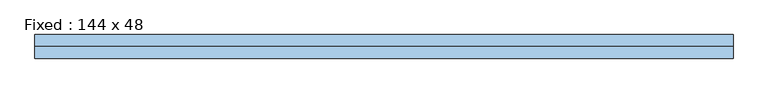
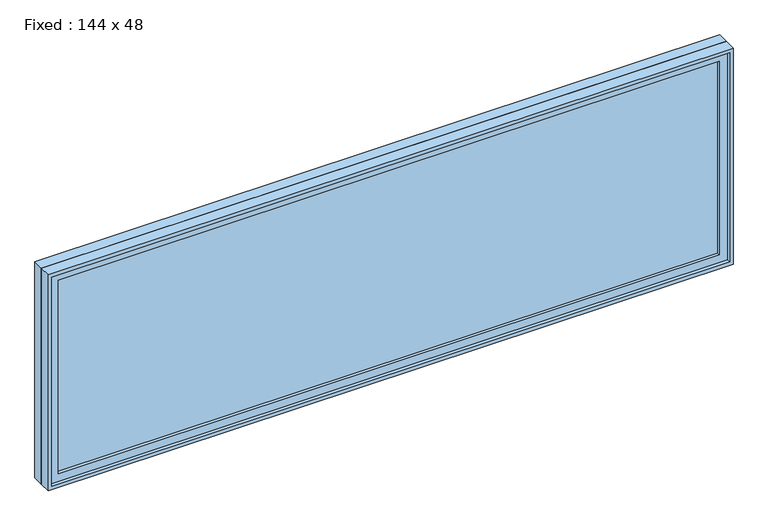
"""IFC4 building model written with IfcOpenShell, lengths in millimetres: window geometry, Fixed : 144 x 48."""

import ifcopenshell
import ifcopenshell.guid

model = None  # the IFC model being written
_history = None  # IfcOwnerHistory: only IFC2X3 demands one
_inside = {}  # id of a spatial element -> (the spatial element, [elements in it])
_under = {}  # id of a project, library or spatial element -> (it, [spatial elements below it])
_declared = {}  # id of a project -> (the project, [libraries it declares])
_typed = {}  # id of a type object -> (the type object, [elements of that type])
_made_of = {}  # id of a material, layer set ... -> (it, [elements and type objects made of it])


def new_model(schema):
    """Start an empty IFC model of exactly this schema.

    Asked for "IFC4X3", IfcOpenShell would pick the latest addendum, in which some entities
    have other attributes; the version numbers below select the first issue.
    IFC2X3 requires an IfcOwnerHistory on every rooted entity: one is made here for all.
    """
    global model, _history
    if schema == "IFC4X3":
        model = ifcopenshell.file(schema_version=(4, 3, 0, 0))
    else:
        model = ifcopenshell.file(schema=schema)
    _inside.clear()
    _under.clear()
    _declared.clear()
    _typed.clear()
    _made_of.clear()
    _history = None
    if model.schema == "IFC2X3":
        org = make("IfcOrganization", Name="unknown")
        user = make(
            "IfcPersonAndOrganization",
            ThePerson=make("IfcPerson", FamilyName="unknown"),
            TheOrganization=org,
        )
        app = make(
            "IfcApplication",
            ApplicationDeveloper=org,
            Version="unknown",
            ApplicationFullName="unknown",
            ApplicationIdentifier="unknown",
        )
        _history = make(
            "IfcOwnerHistory",
            OwningUser=user,
            OwningApplication=app,
            ChangeAction="ADDED",
            CreationDate=0,
        )
    return model


def make(cls, **values):
    """One entity of the class cls with the attributes given. An attribute that is None is left unset."""
    return model.create_entity(
        cls, **{name: value for name, value in values.items() if value is not None}
    )


def rooted(cls, **values):
    """An entity with a GlobalId (a new one), such as an element, a storey or a relation."""
    return make(cls, GlobalId=ifcopenshell.guid.new(), OwnerHistory=_history, **values)


def si_unit(unit_type, name, prefix=None):
    """IfcSIUnit, for example si_unit("LENGTHUNIT", "METRE", prefix="MILLI")."""
    return make("IfcSIUnit", UnitType=unit_type, Prefix=prefix, Name=name)


def assignment(units):
    """IfcUnitAssignment: the units of a project."""
    return None if units is None else make("IfcUnitAssignment", Units=units)


def point(xyz):
    """IfcCartesianPoint."""
    return None if xyz is None else make("IfcCartesianPoint", Coordinates=xyz)


def direction(xyz):
    """IfcDirection."""
    return None if xyz is None else make("IfcDirection", DirectionRatios=xyz)


def frame(location, z_axis=None, x_axis=None):
    """IfcAxis2Placement3D, a coordinate frame: its origin and axes. An axis left out is left unset."""
    return make(
        "IfcAxis2Placement3D",
        Location=point(location),
        Axis=direction(z_axis),
        RefDirection=direction(x_axis),
    )


def origin():
    """The frame at (0, 0, 0) with its axes left unset."""
    return frame((0.0, 0.0, 0.0))


def place(relative_to, where):
    """IfcLocalPlacement: puts the frame where relative to a parent placement (None: the world)."""
    return make(
        "IfcLocalPlacement", PlacementRelTo=relative_to, RelativePlacement=where
    )


def context(
    kind, dimensions, precision=None, world=None, true_north=None, identifier=None
):
    """IfcGeometricRepresentationContext, for example the 3D "Model" context."""
    return make(
        "IfcGeometricRepresentationContext",
        ContextIdentifier=identifier,
        ContextType=kind,
        CoordinateSpaceDimension=dimensions,
        Precision=precision,
        WorldCoordinateSystem=world,
        TrueNorth=true_north,
    )


def project(units=None, contexts=None):
    """IfcProject with its units and contexts."""
    return rooted(
        "IfcProject",
        Name="project",
        RepresentationContexts=contexts,
        UnitsInContext=assignment(units),
    )


def spatial(cls, under=None, at=None, **own):
    """A site, building, storey or space (cls), placed at a placement, below another one or the project."""
    s = rooted(cls, ObjectPlacement=at, **own)
    if under is not None:
        _under.setdefault(under.id(), (under, []))[1].append(s)
    return s


def polyline(points):
    """IfcPolyline through the points."""
    return make("IfcPolyline", Points=[point(p) for p in points])


def outline(outer, holes=None, kind="AREA"):
    """IfcArbitraryClosedProfileDef: a profile drawn as a closed curve; with holes, ...WithVoids."""
    if holes is None:
        return make("IfcArbitraryClosedProfileDef", ProfileType=kind, OuterCurve=outer)
    return make(
        "IfcArbitraryProfileDefWithVoids",
        ProfileType=kind,
        OuterCurve=outer,
        InnerCurves=holes,
    )


def extrude(swept, where, along, depth):
    """IfcExtrudedAreaSolid: the profile swept, set in the frame where, extruded along a direction by depth."""
    return make(
        "IfcExtrudedAreaSolid",
        SweptArea=swept,
        Position=where,
        ExtrudedDirection=direction(along),
        Depth=depth,
    )


def shape(context_of_items, identifier, shape_type, items):
    """IfcShapeRepresentation: the items that make up one representation, for example the "Body"."""
    return make(
        "IfcShapeRepresentation",
        ContextOfItems=context_of_items,
        RepresentationIdentifier=identifier,
        RepresentationType=shape_type,
        Items=items,
    )


def source(mapping_origin, context_of_items, identifier, shape_type, items):
    """IfcRepresentationMap: a shape defined once, which mapped items show again and again."""
    return make(
        "IfcRepresentationMap",
        MappingOrigin=mapping_origin,
        MappedRepresentation=shape(context_of_items, identifier, shape_type, items),
    )


def transform(
    local_origin,
    x_axis=None,
    y_axis=None,
    z_axis=None,
    scale=None,
    scale2=None,
    scale3=None,
    uniform=True,
):
    """IfcCartesianTransformationOperator3D, or its non-uniform kind. x_axis, y_axis, z_axis: its Axis1, 2, 3."""
    if uniform:
        return make(
            "IfcCartesianTransformationOperator3D",
            Axis1=direction(x_axis),
            Axis2=direction(y_axis),
            LocalOrigin=point(local_origin),
            Scale=scale,
            Axis3=direction(z_axis),
        )
    return make(
        "IfcCartesianTransformationOperator3DnonUniform",
        Axis1=direction(x_axis),
        Axis2=direction(y_axis),
        LocalOrigin=point(local_origin),
        Scale=scale,
        Axis3=direction(z_axis),
        Scale2=scale2,
        Scale3=scale3,
    )


def mapped(mapping_source, mapping_target):
    """IfcMappedItem: shows the shape of a source again, moved by a transform."""
    return make(
        "IfcMappedItem", MappingSource=mapping_source, MappingTarget=mapping_target
    )


def made_of(thing, what):
    """Note that an element or type object is made of a material, layer set ...; save() writes the relation."""
    if what is not None:
        _made_of.setdefault(what.id(), (what, []))[1].append(thing)
    return thing


def element(
    cls,
    number,
    at=None,
    inside=None,
    cuts=None,
    type_object=None,
    material=None,
    context=None,
    identifier="Body",
    shape_type=None,
    held_by="IfcProductDefinitionShape",
    body=None,
    shapes=None,
    **own,
):
    """One element of the class cls, such as IfcWall. Its Tag is "e" and its number.

    at: its placement. inside: the storey or other place that contains it. cuts: it is an
    opening in that element (IfcRelVoidsElement). A single representation is given by context,
    identifier, shape_type and body (its items); several are given by shapes. held_by: the class
    of the entity that holds the representations. save() writes the other relations.
    """
    e = rooted(cls, Tag="e%d" % number, ObjectPlacement=at, **own)
    if body is not None:
        shapes = [shape(context, identifier, shape_type, body)]
    if shapes is not None:
        e.Representation = make(held_by, Representations=shapes)
    if inside is not None:
        _inside.setdefault(inside.id(), (inside, []))[1].append(e)
    if cuts is not None:
        rooted(
            "IfcRelVoidsElement", RelatingBuildingElement=cuts, RelatedOpeningElement=e
        )
    if type_object is not None:
        _typed.setdefault(type_object.id(), (type_object, []))[1].append(e)
    return made_of(e, material)


def aggregate(whole, parts):
    """IfcRelAggregates: a whole, such as a stair, and the parts it consists of."""
    return rooted("IfcRelAggregates", RelatingObject=whole, RelatedObjects=parts)


def save(model, path):
    """Write the relations noted so far, then the file.

    IfcRelAggregates (storeys below a building ...), IfcRelContainedInSpatialStructure (elements
    in a storey), IfcRelDefinesByType, IfcRelAssociatesMaterial and IfcRelDeclares: one each for
    every whole, place, type object, material and project.
    """
    for whole, parts in _under.values():
        aggregate(whole, parts)
    for where, things in _inside.values():
        rooted(
            "IfcRelContainedInSpatialStructure",
            RelatedElements=things,
            RelatingStructure=where,
        )
    for kind, things in _typed.values():
        rooted("IfcRelDefinesByType", RelatedObjects=things, RelatingType=kind)
    for what, things in _made_of.values():
        rooted("IfcRelAssociatesMaterial", RelatedObjects=things, RelatingMaterial=what)
    for by, libraries in _declared.values():
        rooted("IfcRelDeclares", RelatingContext=by, RelatedDefinitions=libraries)
    model.write(path)


def fixed_144_x_48_29d34a77(model_context):
    return source(origin(), model_context, "Body", "SweptSolid", [
        extrude(outline(polyline([(1727.2, -14.2875), (1727.2, -26.9875), (-1803.4, -26.9875), (-1803.4, -14.2875), (1727.2, -14.2875)])), frame((0.0, 0.0, 977.9), z_axis=(0.0, 0.0, 1.0), x_axis=(1.0, 0.0, 0.0)), (0.0, 0.0, 1.0), 1092.2),
        extrude(outline(polyline([(2114.55, -1847.85), (933.45, -1847.85), (933.45, 1771.65), (2114.55, 1771.65), (2114.55, -1847.85)]), holes=[polyline([(2070.1, -1803.4), (2070.1, 1727.2), (977.9, 1727.2), (977.9, -1803.4), (2070.1, -1803.4)])]), frame((0.0, -42.8625, 0.0), z_axis=(0.0, 1.0, 0.0), x_axis=(0.0, 0.0, 1.0)), (0.0, 0.0, 1.0), 44.45),
        extrude(outline(polyline([(2133.6, -1866.9), (914.4, -1866.9), (914.4, 1790.7), (2133.6, 1790.7), (2133.6, -1866.9)]), holes=[polyline([(2101.85, -1835.15), (2101.85, 1758.95), (946.15, 1758.95), (946.15, -1835.15), (2101.85, -1835.15)])]), frame((0.0, 1.5875, 0.0), z_axis=(0.0, 1.0, 0.0), x_axis=(0.0, 0.0, 1.0)), (0.0, 0.0, 1.0), 60.325),
        extrude(outline(polyline([(2133.6, 1790.7), (2133.6, -1866.9), (914.4, -1866.9), (914.4, 1790.7), (2133.6, 1790.7)]), holes=[polyline([(2114.55, 1771.65), (933.45, 1771.65), (933.45, -1847.85), (2114.55, -1847.85), (2114.55, 1771.65)])]), frame((0.0, -61.9125, 0.0), z_axis=(0.0, 1.0, 0.0), x_axis=(0.0, 0.0, 1.0)), (0.0, 0.0, 1.0), 63.5),
    ])


if __name__ == "__main__":
    model = new_model("IFC4")
    model_context = context("Model", 3, world=origin())
    ifc_project = project(units=[si_unit("LENGTHUNIT", "METRE", prefix="MILLI")], contexts=[model_context])
    site = spatial("IfcSite", under=ifc_project)
    building = spatial("IfcBuilding", under=site)
    placement = place(None, origin())
    fixed_144_x_48_shape = fixed_144_x_48_29d34a77(model_context)
    element("IfcWindow", 1, ObjectType="Fixed : 144 x 48", at=placement, inside=building, context=model_context, shape_type="MappedRepresentation", body=[
        mapped(fixed_144_x_48_shape, transform((0.0, 0.0, 0.0), x_axis=(1.0, 0.0, 0.0), y_axis=(0.0, 1.0, 0.0), z_axis=(0.0, 0.0, 1.0))),
    ])
    save(model, "model.ifc")

# Revit data of these elements
# Type "Fixed : 144 x 48"
#   Type Mark = "11"
#   Assembly Code = "B2020100"
#   Height = 4' - 0"
#   Default Sill Height = 3' - 0"
#   Width = 12' - 0"
#   Window Inset = 0' - 0 3/4"
#   Glass Pane Material = Glass
#   Sash Material = Sash
#   Wall Closure = (empty or 0)
# Element 1 (IfcWindow, "Fixed : 144 x 48")
#   Materials on its faces: "Sash", "Glass"
# Materials
#   "Glass": class "Glass", colour RGB 0 128 192, transparency 0.75
#   "Sash": class "Wood", colour RGB 224 178 126, transparency 0
